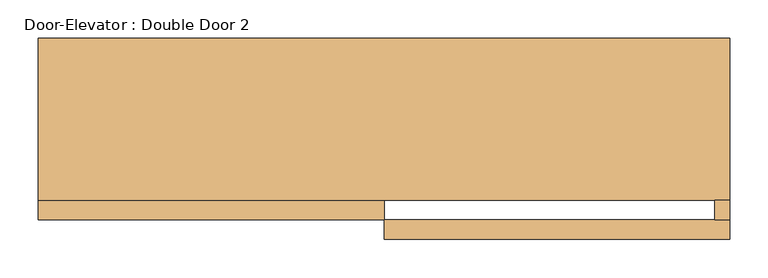
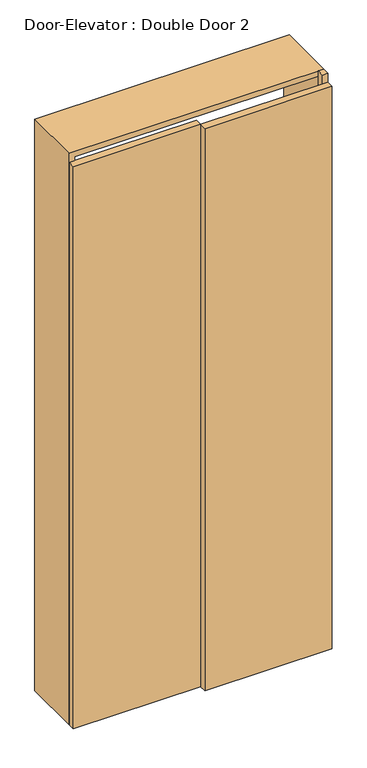
"""IFC4 building model written with IfcOpenShell, lengths in millimetres: door geometry, Door-Elevator : Double Door 2."""

from ifc_helpers import new_model, si_unit, frame, origin, origin_with_axes, place, context, project, spatial, polyline, outline, extrude, source, transform, mapped, element, save


def door_elevator_double_door_2_46fda4f0(model_context):
    return source(origin(), model_context, "Body", "SweptSolid", [
        extrude(outline(polyline([(450.0, -147.15), (450.0, -172.55), (0.0, -172.55), (0.0, -147.15), (450.0, -147.15)])), origin_with_axes(), (0.0, 0.0, 1.0), 2100.0),
        extrude(outline(polyline([(0.0, -121.75), (0.0, -147.15), (-450.0, -147.15), (-450.0, -121.75), (0.0, -121.75)])), origin_with_axes(), (0.0, 0.0, 1.0), 2100.0),
        extrude(outline(polyline([(450.0, -121.75), (450.0, -147.15), (430.95, -147.15), (430.95, -121.75), (450.0, -121.75)])), origin_with_axes(), (0.0, 0.0, 1.0), 2133.6),
        extrude(outline(polyline([(0.0, -430.95), (2114.55, -430.95), (2114.55, 430.95), (0.0, 430.95), (0.0, 450.0), (2133.6, 450.0), (2133.6, -450.0), (0.0, -450.0), (0.0, -430.95)])), frame((0.0, -121.75, 0.0), z_axis=(0.0, 1.0, 0.0), x_axis=(0.0, 0.0, 1.0)), (0.0, 0.0, 1.0), 210.65),
    ])


if __name__ == "__main__":
    model = new_model("IFC4")
    model_context = context("Model", 3, world=origin())
    ifc_project = project(units=[si_unit("LENGTHUNIT", "METRE", prefix="MILLI")], contexts=[model_context])
    site = spatial("IfcSite", under=ifc_project)
    building = spatial("IfcBuilding", under=site)
    placement = place(None, origin())
    door_elevator_double_door_2_shape = door_elevator_double_door_2_46fda4f0(model_context)
    element("IfcDoor", 1, ObjectType="Door-Elevator : Double Door 2", at=placement, inside=building, context=model_context, shape_type="MappedRepresentation", body=[
        mapped(door_elevator_double_door_2_shape, transform((0.0, 0.0, 0.0), x_axis=(1.0, 0.0, 0.0), y_axis=(0.0, 1.0, 0.0), z_axis=(0.0, 0.0, 1.0))),
    ])
    save(model, "model.ifc")

# Revit data of these elements
# Type "Door-Elevator : Double Door 2"
#   Type Mark = "EX1-59"
#   P_WWSKU = ""
#   Filter Visibiilty = "Existing Elevator"
#   Analytic Construction = "<None>"
#   Trim Projection = 12.7 mm
#   Thickness = 25.4 mm
#   Height = 2100 mm
#   Trim Width = 19.05 mm
#   Width = 900 mm
#   Door_Quad = 225 mm
#   Door_Double = 450 mm
#   Cab Width = 1828.8 mm
#   Cab Offset [instance default] = 0 mm
#   Cab Depth = 1828.8 mm
#   _factor4 = 4
#   _factor2 = 2
#   WW-HardwareSet [instance default] = 0
#   Simple Plan = yes
#   Quad = no
#   Plan Lines [instance default] = yes
#   Double = yes
#   Panel Type = element 9002524
#   Type Comments = ""
#   Keynote = ""
#   Function = (empty or 0)
#   Wall Closure = (empty or 0)
#   Assembly Code = ""
# Element 1 (IfcDoor, "Door-Elevator : Double Door 2")
#   Materials on its faces: "WW-EC-RGB-White"
# Materials
#   "WW-EC-RGB-White": class "Generic", colour RGB 255 255 255, transparency 0, Comments = "If region requests off-white, swith asset color to RGB 231-228-220", Description = "Generic Color", Cost = 0
